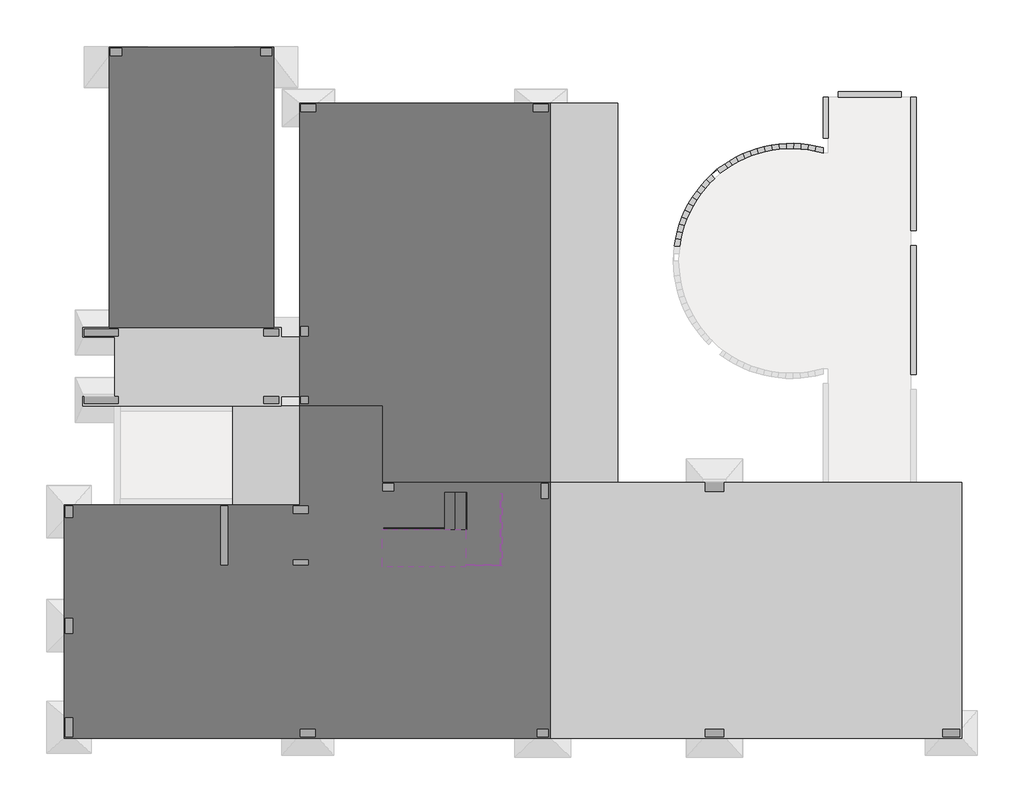
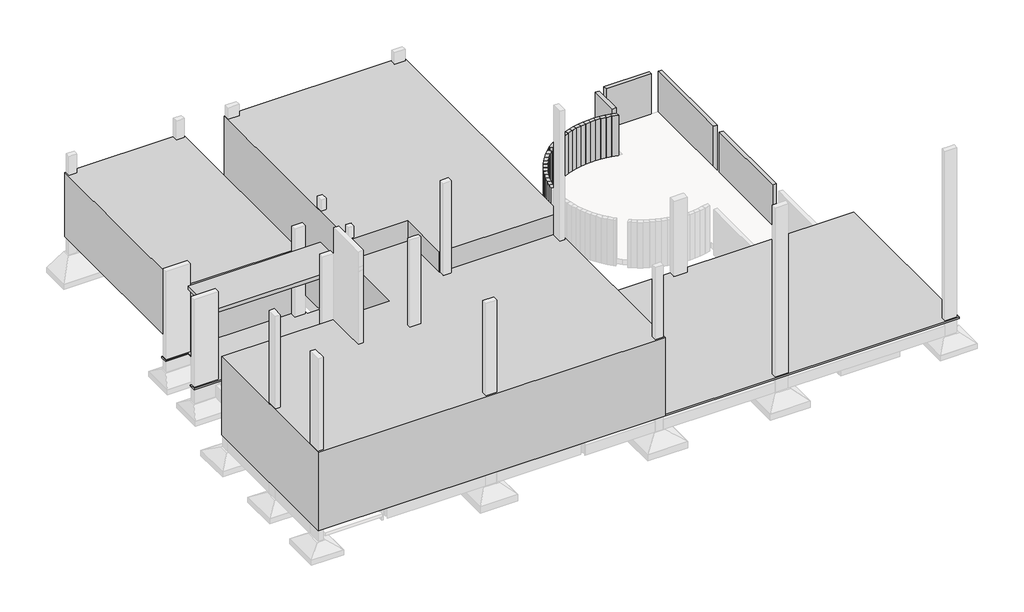
# One storey, part 4 of 4: 29 beams, 7 proxies, 6 railings, 2 stair flights, 1 slab.
# Revit data of these elements (continued)
# Type "ML_Guarda_corpo lance1 : ML_Guarda_corpo lance" (continued)
#   ME_Material Tipo Vidro [instance default] = .VIDRO GENÉRICO
# Element 1 (IfcBeam, "TQS - Viga retangular : 14.0 x 180.0")
#   Uso = "ESTRUTURA"
#   Titulo = "VP1"
#   Chave = "-983"
#   Tipo Elemento = "Viga"
#   SHA1 = "70CFAD44B8F4F6228BE95B7E8E7C3E9A2DD88366"
#   Revisão = ""
#   Tipo de carga = ""
#   Divisor de flexao = ""
#   Secao = ""
#   Configuracao = ""
#   Angulo (graus) = ""
#   Detalhamento = ""
#   Casos de vento manual = ""
#   Tipo = ""
#   Alcas = ""
#   Furos = ""
#   Pino = ""
#   Distribuicao = ""
#   Solidarizado = ""
#   Solidarizar na montagem = ""
#   Unir com o próximo = ""
#   Grupo pre moldado = ""
#   Verificado = ""
#   Concreto C = ""
#   Taxa de armadura (kgf/m³) = 0
#   Carga (tf/m²) = 0
#   Carga (tf/m) = 0
#   Carga (tf) = 0
#   Altura = 1.80 m
#   Rebaixo = 0.15 m
#   Largura = 0.14 m
#   Distancia a face = 0.00 m
#   Distancia ao eixo = 0.00 m
#   Altura gerber esquerda = 0.00 m
#   Largura gerber esquerda = 0.00 m
#   Altura gerber direita = 0.00 m
#   Largura gerber direita = 0.00 m
#   Resultado de Ensaios fck (MPa) = 0
#   Unique TQS ID = -983
#   Principal = yes
#   Structural Material = none
#   Phase Created = CC_AP/ESTR
# Element 2 (IfcBeam, "TQS - Viga retangular : 14.0 x 180.0")
#   Uso = "ESTRUTURA"
#   Titulo = "VP6"
#   Chave = "-1015"
#   Tipo Elemento = "Viga"
#   SHA1 = "4E9806910888EA421A8E9B5F41FC3E19263D6A9E"
#   Revisão = ""
#   Tipo de carga = ""
#   Divisor de flexao = ""
#   Secao = ""
#   Configuracao = ""
#   Angulo (graus) = ""
#   Detalhamento = ""
#   Casos de vento manual = ""
#   Tipo = ""
#   Alcas = ""
#   Furos = ""
#   Pino = ""
#   Distribuicao = ""
#   Solidarizado = ""
#   Solidarizar na montagem = ""
#   Unir com o próximo = ""
#   Grupo pre moldado = ""
#   Verificado = ""
#   Concreto C = ""
#   Taxa de armadura (kgf/m³) = 0
#   Carga (tf/m²) = 0
#   Carga (tf/m) = 0
#   Carga (tf) = 0
#   Altura = 1.80 m
#   Rebaixo = 0.15 m
#   Largura = 0.14 m
#   Distancia a face = 0.00 m
#   Distancia ao eixo = 0.00 m
#   Altura gerber esquerda = 0.00 m
#   Largura gerber esquerda = 0.00 m
#   Altura gerber direita = 0.00 m
#   Largura gerber direita = 0.00 m
#   Resultado de Ensaios fck (MPa) = 0
#   Unique TQS ID = -1015
#   Principal = yes
#   Structural Material = none
#   Phase Created = CC_AP/ESTR
# Element 3 (IfcBeam, "TQS - Viga retangular : 14.0 x 180.0")
#   Uso = "ESTRUTURA"
#   Titulo = "VP6"
#   Chave = "-1016"
#   Tipo Elemento = "Viga"
#   SHA1 = "01F1283C1B0C380DFDB901244E097327FB4B1C7E"
#   Revisão = ""
#   Tipo de carga = ""
#   Divisor de flexao = ""
#   Secao = ""
#   Configuracao = ""
#   Angulo (graus) = ""
#   Detalhamento = ""
#   Casos de vento manual = ""
#   Tipo = ""
#   Alcas = ""
#   Furos = ""
#   Pino = ""
#   Distribuicao = ""
#   Solidarizado = ""
#   Solidarizar na montagem = ""
#   Unir com o próximo = ""
#   Grupo pre moldado = ""
#   Verificado = ""
#   Concreto C = ""
#   Taxa de armadura (kgf/m³) = 0
#   Carga (tf/m²) = 0
#   Carga (tf/m) = 0
#   Carga (tf) = 0
#   Altura = 1.80 m
#   Rebaixo = 0.15 m
#   Largura = 0.14 m
#   Distancia a face = 0.00 m
#   Distancia ao eixo = 0.00 m
#   Altura gerber esquerda = 0.00 m
#   Largura gerber esquerda = 0.00 m
#   Altura gerber direita = 0.00 m
#   Largura gerber direita = 0.00 m
#   Resultado de Ensaios fck (MPa) = 0
#   Unique TQS ID = -1016
#   Principal = yes
#   Structural Material = none
#   Phase Created = CC_AP/ESTR
# Element 4 (IfcBeam, "TQS - Viga retangular : 14.0 x 180.0")
#   Uso = "ESTRUTURA"
#   Titulo = "VP6"
#   Chave = "-1017"
#   Tipo Elemento = "Viga"
#   SHA1 = "22C0BDACD46D49F6E4190D80621E2138C68CD36C"
#   Revisão = ""
#   Tipo de carga = ""
#   Divisor de flexao = ""
#   Secao = ""
#   Configuracao = ""
#   Angulo (graus) = ""
#   Detalhamento = ""
#   Casos de vento manual = ""
#   Tipo = ""
#   Alcas = ""
#   Furos = ""
#   Pino = ""
#   Distribuicao = ""
#   Solidarizado = ""
#   Solidarizar na montagem = ""
#   Unir com o próximo = ""
#   Grupo pre moldado = ""
#   Verificado = ""
#   Concreto C = ""
#   Taxa de armadura (kgf/m³) = 0
#   Carga (tf/m²) = 0
#   Carga (tf/m) = 0
#   Carga (tf) = 0
#   Altura = 1.80 m
#   Rebaixo = 0.15 m
#   Largura = 0.14 m
#   Distancia a face = 0.00 m
#   Distancia ao eixo = 0.00 m
#   Altura gerber esquerda = 0.00 m
#   Largura gerber esquerda = 0.00 m
#   Altura gerber direita = 0.00 m
#   Largura gerber direita = 0.00 m
#   Resultado de Ensaios fck (MPa) = 0
#   Unique TQS ID = -1017
#   Principal = yes
#   Structural Material = none
#   Phase Created = CC_AP/ESTR
# Element 5 (IfcBeam, "TQS - Viga retangular : 14.0 x 180.0")
#   Uso = "ESTRUTURA"
#   Titulo = "VP6"
#   Chave = "-1018"
#   Tipo Elemento = "Viga"
#   SHA1 = "D04A2C827C3C8BC1853343DA7F217DB9B9B2F05D"
#   Revisão = ""
#   Tipo de carga = ""
#   Divisor de flexao = ""
#   Secao = ""
#   Configuracao = ""
#   Angulo (graus) = ""
#   Detalhamento = ""
#   Casos de vento manual = ""
#   Tipo = ""
#   Alcas = ""
#   Furos = ""
#   Pino = ""
#   Distribuicao = ""
#   Solidarizado = ""
#   Solidarizar na montagem = ""
#   Unir com o próximo = ""
#   Grupo pre moldado = ""
#   Verificado = ""
#   Concreto C = ""
#   Taxa de armadura (kgf/m³) = 0
#   Carga (tf/m²) = 0
#   Carga (tf/m) = 0
#   Carga (tf) = 0
#   Altura = 1.80 m
#   Rebaixo = 0.15 m
#   Largura = 0.14 m
#   Distancia a face = 0.00 m
#   Distancia ao eixo = 0.00 m
#   Altura gerber esquerda = 0.00 m
#   Largura gerber esquerda = 0.00 m
#   Altura gerber direita = 0.00 m
#   Largura gerber direita = 0.00 m
#   Resultado de Ensaios fck (MPa) = 0
#   Unique TQS ID = -1018
#   Principal = yes
#   Structural Material = none
#   Phase Created = CC_AP/ESTR
# Element 6 (IfcBeam, "TQS - Viga retangular : 14.0 x 180.0")
#   Uso = "ESTRUTURA"
#   Titulo = "VP6"
#   Chave = "-1019"
#   Tipo Elemento = "Viga"
#   SHA1 = "0D182E2612785E293A5A4969EBA47990CD3E9117"
#   Revisão = ""
#   Tipo de carga = ""
#   Divisor de flexao = ""
#   Secao = ""
#   Configuracao = ""
#   Angulo (graus) = ""
#   Detalhamento = ""
#   Casos de vento manual = ""
#   Tipo = ""
#   Alcas = ""
#   Furos = ""
#   Pino = ""
#   Distribuicao = ""
#   Solidarizado = ""
#   Solidarizar na montagem = ""
#   Unir com o próximo = ""
#   Grupo pre moldado = ""
#   Verificado = ""
#   Concreto C = ""
#   Taxa de armadura (kgf/m³) = 0
#   Carga (tf/m²) = 0
#   Carga (tf/m) = 0
#   Carga (tf) = 0
#   Altura = 1.80 m
#   Rebaixo = 0.15 m
#   Largura = 0.14 m
#   Distancia a face = 0.00 m
#   Distancia ao eixo = 0.00 m
#   Altura gerber esquerda = 0.00 m
#   Largura gerber esquerda = 0.00 m
#   Altura gerber direita = 0.00 m
#   Largura gerber direita = 0.00 m
#   Resultado de Ensaios fck (MPa) = 0
#   Unique TQS ID = -1019
#   Principal = yes
#   Structural Material = none
#   Phase Created = CC_AP/ESTR
# Element 7 (IfcBeam, "TQS - Viga retangular : 14.0 x 180.0")
#   Uso = "ESTRUTURA"
#   Titulo = "VP6"
#   Chave = "-1020"
#   Tipo Elemento = "Viga"
#   SHA1 = "8A5DF36B72EBE22F2A453D6F9BADDE3EA3E2A9B4"
#   Revisão = ""
#   Tipo de carga = ""
#   Divisor de flexao = ""
#   Secao = ""
#   Configuracao = ""
#   Angulo (graus) = ""
#   Detalhamento = ""
#   Casos de vento manual = ""
#   Tipo = ""
#   Alcas = ""
#   Furos = ""
#   Pino = ""
#   Distribuicao = ""
#   Solidarizado = ""
#   Solidarizar na montagem = ""
#   Unir com o próximo = ""
#   Grupo pre moldado = ""
#   Verificado = ""
#   Concreto C = ""
#   Taxa de armadura (kgf/m³) = 0
#   Carga (tf/m²) = 0
#   Carga (tf/m) = 0
#   Carga (tf) = 0
#   Altura = 1.80 m
#   Rebaixo = 0.15 m
#   Largura = 0.14 m
#   Distancia a face = 0.00 m
#   Distancia ao eixo = 0.00 m
#   Altura gerber esquerda = 0.00 m
#   Largura gerber esquerda = 0.00 m
#   Altura gerber direita = 0.00 m
#   Largura gerber direita = 0.00 m
#   Resultado de Ensaios fck (MPa) = 0
#   Unique TQS ID = -1020
#   Principal = yes
#   Structural Material = none
#   Phase Created = CC_AP/ESTR
# Element 8 (IfcBeam, "TQS - Viga retangular : 14.0 x 180.0")
#   Uso = "ESTRUTURA"
#   Titulo = "VP6"
#   Chave = "-1021"
#   Tipo Elemento = "Viga"
#   SHA1 = "E996D88AC41B572457E87FBE2BFAA83C91B590B4"
#   Revisão = ""
#   Tipo de carga = ""
#   Divisor de flexao = ""
#   Secao = ""
#   Configuracao = ""
#   Angulo (graus) = ""
#   Detalhamento = ""
#   Casos de vento manual = ""
#   Tipo = ""
#   Alcas = ""
#   Furos = ""
#   Pino = ""
#   Distribuicao = ""
#   Solidarizado = ""
#   Solidarizar na montagem = ""
#   Unir com o próximo = ""
#   Grupo pre moldado = ""
#   Verificado = ""
#   Concreto C = ""
#   Taxa de armadura (kgf/m³) = 0
#   Carga (tf/m²) = 0
#   Carga (tf/m) = 0
#   Carga (tf) = 0
#   Altura = 1.80 m
#   Rebaixo = 0.15 m
#   Largura = 0.14 m
#   Distancia a face = 0.00 m
#   Distancia ao eixo = 0.00 m
#   Altura gerber esquerda = 0.00 m
#   Largura gerber esquerda = 0.00 m
#   Altura gerber direita = 0.00 m
#   Largura gerber direita = 0.00 m
#   Resultado de Ensaios fck (MPa) = 0
#   Unique TQS ID = -1021
#   Principal = yes
#   Structural Material = none
#   Phase Created = CC_AP/ESTR
# Element 9 (IfcBeam, "TQS - Viga retangular : 14.0 x 180.0")
#   Uso = "ESTRUTURA"
#   Titulo = "VP6"
#   Chave = "-1022"
#   Tipo Elemento = "Viga"
#   SHA1 = "0B33ED0C5CE953F65B7DD0F51C60662F46F82846"
#   Revisão = ""
#   Tipo de carga = ""
#   Divisor de flexao = ""
#   Secao = ""
#   Configuracao = ""
#   Angulo (graus) = ""
#   Detalhamento = ""
#   Casos de vento manual = ""
#   Tipo = ""
#   Alcas = ""
#   Furos = ""
#   Pino = ""
#   Distribuicao = ""
#   Solidarizado = ""
#   Solidarizar na montagem = ""
#   Unir com o próximo = ""
#   Grupo pre moldado = ""
#   Verificado = ""
#   Concreto C = ""
#   Taxa de armadura (kgf/m³) = 0
#   Carga (tf/m²) = 0
#   Carga (tf/m) = 0
#   Carga (tf) = 0
#   Altura = 1.80 m
#   Rebaixo = 0.15 m
#   Largura = 0.14 m
#   Distancia a face = 0.00 m
#   Distancia ao eixo = 0.00 m
#   Altura gerber esquerda = 0.00 m
#   Largura gerber esquerda = 0.00 m
#   Altura gerber direita = 0.00 m
#   Largura gerber direita = 0.00 m
#   Resultado de Ensaios fck (MPa) = 0
#   Unique TQS ID = -1022
#   Principal = yes
#   Structural Material = none
#   Phase Created = CC_AP/ESTR
# Element 10 (IfcBeam, "TQS - Viga retangular : 14.0 x 180.0")
#   Uso = "ESTRUTURA"
#   Titulo = "VP6"
#   Chave = "-1023"
#   Tipo Elemento = "Viga"
#   SHA1 = "7A0208B774D9472BDEB9F4D9C600465610707295"
#   Revisão = ""
#   Tipo de carga = ""
#   Divisor de flexao = ""
#   Secao = ""
#   Configuracao = ""
#   Angulo (graus) = ""
#   Detalhamento = ""
#   Casos de vento manual = ""
#   Tipo = ""
#   Alcas = ""
#   Furos = ""
#   Pino = ""
#   Distribuicao = ""
#   Solidarizado = ""
#   Solidarizar na montagem = ""
#   Unir com o próximo = ""
#   Grupo pre moldado = ""
#   Verificado = ""
#   Concreto C = ""
#   Taxa de armadura (kgf/m³) = 0
#   Carga (tf/m²) = 0
#   Carga (tf/m) = 0
#   Carga (tf) = 0
#   Altura = 1.80 m
#   Rebaixo = 0.15 m
#   Largura = 0.14 m
#   Distancia a face = 0.00 m
#   Distancia ao eixo = 0.00 m
#   Altura gerber esquerda = 0.00 m
#   Largura gerber esquerda = 0.00 m
#   Altura gerber direita = 0.00 m
#   Largura gerber direita = 0.00 m
#   Resultado de Ensaios fck (MPa) = 0
#   Unique TQS ID = -1023
#   Principal = yes
#   Structural Material = none
#   Phase Created = CC_AP/ESTR
# Element 11 (IfcBeam, "TQS - Viga retangular : 14.0 x 180.0")
#   Uso = "ESTRUTURA"
#   Titulo = "VP6"
#   Chave = "-1024"
#   Tipo Elemento = "Viga"
#   SHA1 = "84182F31E964F02A91D7472A67EEC15D959BEA6F"
#   Revisão = ""
#   Tipo de carga = ""
#   Divisor de flexao = ""
#   Secao = ""
#   Configuracao = ""
#   Angulo (graus) = ""
#   Detalhamento = ""
#   Casos de vento manual = ""
#   Tipo = ""
#   Alcas = ""
#   Furos = ""
#   Pino = ""
#   Distribuicao = ""
#   Solidarizado = ""
#   Solidarizar na montagem = ""
#   Unir com o próximo = ""
#   Grupo pre moldado = ""
#   Verificado = ""
#   Concreto C = ""
#   Taxa de armadura (kgf/m³) = 0
#   Carga (tf/m²) = 0
#   Carga (tf/m) = 0
#   Carga (tf) = 0
#   Altura = 1.80 m
#   Rebaixo = 0.15 m
#   Largura = 0.14 m
#   Distancia a face = 0.00 m
#   Distancia ao eixo = 0.00 m
#   Altura gerber esquerda = 0.00 m
#   Largura gerber esquerda = 0.00 m
#   Altura gerber direita = 0.00 m
#   Largura gerber direita = 0.00 m
#   Resultado de Ensaios fck (MPa) = 0
#   Unique TQS ID = -1024
#   Principal = yes
#   Structural Material = none
#   Phase Created = CC_AP/ESTR
# Element 12 (IfcBeam, "TQS - Viga retangular : 14.0 x 180.0")
#   Uso = "ESTRUTURA"
#   Titulo = "VP6"
#   Chave = "-1025"
#   Tipo Elemento = "Viga"
#   SHA1 = "018AD11D8442C61DF0F4C6D5519537CB9DF1785E"
#   Revisão = ""
#   Tipo de carga = ""
#   Divisor de flexao = ""
#   Secao = ""
#   Configuracao = ""
#   Angulo (graus) = ""
#   Detalhamento = ""
#   Casos de vento manual = ""
#   Tipo = ""
#   Alcas = ""
#   Furos = ""
#   Pino = ""
#   Distribuicao = ""
#   Solidarizado = ""
#   Solidarizar na montagem = ""
#   Unir com o próximo = ""
#   Grupo pre moldado = ""
#   Verificado = ""
#   Concreto C = ""
#   Taxa de armadura (kgf/m³) = 0
#   Carga (tf/m²) = 0
#   Carga (tf/m) = 0
#   Carga (tf) = 0
#   Altura = 1.80 m
#   Rebaixo = 0.15 m
#   Largura = 0.14 m
#   Distancia a face = 0.00 m
#   Distancia ao eixo = 0.00 m
#   Altura gerber esquerda = 0.00 m
#   Largura gerber esquerda = 0.00 m
#   Altura gerber direita = 0.00 m
#   Largura gerber direita = 0.00 m
#   Resultado de Ensaios fck (MPa) = 0
#   Unique TQS ID = -1025
#   Principal = yes
#   Structural Material = none
#   Phase Created = CC_AP/ESTR
# Element 13 (IfcBeam, "TQS - Viga retangular : 14.0 x 180.0")
#   Uso = "ESTRUTURA"
#   Titulo = "VP7"
#   Chave = "-1026"
#   Tipo Elemento = "Viga"
#   SHA1 = "EE0903180FC4F74752EE8D351596400DB6C4E3D3"
#   Revisão = ""
#   Tipo de carga = ""
#   Divisor de flexao = ""
#   Secao = ""
#   Configuracao = ""
#   Angulo (graus) = ""
#   Detalhamento = ""
#   Casos de vento manual = ""
#   Tipo = ""
#   Alcas = ""
#   Furos = ""
#   Pino = ""
#   Distribuicao = ""
#   Solidarizado = ""
#   Solidarizar na montagem = ""
#   Unir com o próximo = ""
#   Grupo pre moldado = ""
#   Verificado = ""
#   Concreto C = ""
#   Taxa de armadura (kgf/m³) = 0
#   Carga (tf/m²) = 0
#   Carga (tf/m) = 0
#   Carga (tf) = 0
#   Altura = 1.80 m
#   Rebaixo = 0.15 m
#   Largura = 0.14 m
#   Distancia a face = 0.00 m
#   Distancia ao eixo = 0.00 m
#   Altura gerber esquerda = 0.00 m
#   Largura gerber esquerda = 0.00 m
#   Altura gerber direita = 0.00 m
#   Largura gerber direita = 0.00 m
#   Resultado de Ensaios fck (MPa) = 0
#   Unique TQS ID = -1026
#   Principal = yes
#   Structural Material = none
#   Phase Created = CC_AP/ESTR
# Element 14 (IfcBeam, "TQS - Viga retangular : 14.0 x 180.0")
#   Uso = "ESTRUTURA"
#   Titulo = "VP7"
#   Chave = "-1027"
#   Tipo Elemento = "Viga"
#   SHA1 = "9C0E264E63AB224DB050780EBEBCCF0090D66D0A"
#   Revisão = ""
#   Tipo de carga = ""
#   Divisor de flexao = ""
#   Secao = ""
#   Configuracao = ""
#   Angulo (graus) = ""
#   Detalhamento = ""
#   Casos de vento manual = ""
#   Tipo = ""
#   Alcas = ""
#   Furos = ""
#   Pino = ""
#   Distribuicao = ""
#   Solidarizado = ""
#   Solidarizar na montagem = ""
#   Unir com o próximo = ""
#   Grupo pre moldado = ""
#   Verificado = ""
#   Concreto C = ""
#   Taxa de armadura (kgf/m³) = 0
#   Carga (tf/m²) = 0
#   Carga (tf/m) = 0
#   Carga (tf) = 0
#   Altura = 1.80 m
#   Rebaixo = 0.15 m
#   Largura = 0.14 m
#   Distancia a face = 0.00 m
#   Distancia ao eixo = 0.00 m
#   Altura gerber esquerda = 0.00 m
#   Largura gerber esquerda = 0.00 m
#   Altura gerber direita = 0.00 m
#   Largura gerber direita = 0.00 m
#   Resultado de Ensaios fck (MPa) = 0
#   Unique TQS ID = -1027
#   Principal = yes
#   Structural Material = none
#   Phase Created = CC_AP/ESTR
# Element 15 (IfcBeam, "TQS - Viga retangular : 14.0 x 180.0")
#   Uso = "ESTRUTURA"
#   Titulo = "VP7"
#   Chave = "-1028"
#   Tipo Elemento = "Viga"
#   SHA1 = "6E997BB4E590CA8C89FDA8B6D3FF6154DFE7002F"
#   Revisão = ""
#   Tipo de carga = ""
#   Divisor de flexao = ""
#   Secao = ""
#   Configuracao = ""
#   Angulo (graus) = ""
#   Detalhamento = ""
#   Casos de vento manual = ""
#   Tipo = ""
#   Alcas = ""
#   Furos = ""
#   Pino = ""
#   Distribuicao = ""
#   Solidarizado = ""
#   Solidarizar na montagem = ""
#   Unir com o próximo = ""
#   Grupo pre moldado = ""
#   Verificado = ""
#   Concreto C = ""
#   Taxa de armadura (kgf/m³) = 0
#   Carga (tf/m²) = 0
#   Carga (tf/m) = 0
#   Carga (tf) = 0
#   Altura = 1.80 m
#   Rebaixo = 0.15 m
#   Largura = 0.14 m
#   Distancia a face = 0.00 m
#   Distancia ao eixo = 0.00 m
#   Altura gerber esquerda = 0.00 m
#   Largura gerber esquerda = 0.00 m
#   Altura gerber direita = 0.00 m
#   Largura gerber direita = 0.00 m
#   Resultado de Ensaios fck (MPa) = 0
#   Unique TQS ID = -1028
#   Principal = yes
#   Structural Material = none
#   Phase Created = CC_AP/ESTR
# Element 16 (IfcBeam, "TQS - Viga retangular : 14.0 x 180.0")
#   Uso = "ESTRUTURA"
#   Titulo = "VP7"
#   Chave = "-1029"
#   Tipo Elemento = "Viga"
#   SHA1 = "7DDF74561A6D880C43286526A234CDA9ECB81B66"
#   Revisão = ""
#   Tipo de carga = ""
#   Divisor de flexao = ""
#   Secao = ""
#   Configuracao = ""
#   Angulo (graus) = ""
#   Detalhamento = ""
#   Casos de vento manual = ""
#   Tipo = ""
#   Alcas = ""
#   Furos = ""
#   Pino = ""
#   Distribuicao = ""
#   Solidarizado = ""
#   Solidarizar na montagem = ""
#   Unir com o próximo = ""
#   Grupo pre moldado = ""
#   Verificado = ""
#   Concreto C = ""
#   Taxa de armadura (kgf/m³) = 0
#   Carga (tf/m²) = 0
#   Carga (tf/m) = 0
#   Carga (tf) = 0
#   Altura = 1.80 m
#   Rebaixo = 0.15 m
#   Largura = 0.14 m
#   Distancia a face = 0.00 m
#   Distancia ao eixo = 0.00 m
#   Altura gerber esquerda = 0.00 m
#   Largura gerber esquerda = 0.00 m
#   Altura gerber direita = 0.00 m
#   Largura gerber direita = 0.00 m
#   Resultado de Ensaios fck (MPa) = 0
#   Unique TQS ID = -1029
#   Principal = yes
#   Structural Material = none
#   Phase Created = CC_AP/ESTR
# Element 17 (IfcBeam, "TQS - Viga retangular : 14.0 x 180.0")
#   Uso = "ESTRUTURA"
#   Titulo = "VP7"
#   Chave = "-1030"
#   Tipo Elemento = "Viga"
#   SHA1 = "2D411C14CB7CE55D4F1E0A23351751B1C30F9CC4"
#   Revisão = ""
#   Tipo de carga = ""
#   Divisor de flexao = ""
#   Secao = ""
#   Configuracao = ""
#   Angulo (graus) = ""
#   Detalhamento = ""
#   Casos de vento manual = ""
#   Tipo = ""
#   Alcas = ""
#   Furos = ""
#   Pino = ""
#   Distribuicao = ""
#   Solidarizado = ""
#   Solidarizar na montagem = ""
#   Unir com o próximo = ""
#   Grupo pre moldado = ""
#   Verificado = ""
#   Concreto C = ""
#   Taxa de armadura (kgf/m³) = 0
#   Carga (tf/m²) = 0
#   Carga (tf/m) = 0
#   Carga (tf) = 0
#   Altura = 1.80 m
#   Rebaixo = 0.15 m
#   Largura = 0.14 m
#   Distancia a face = 0.00 m
#   Distancia ao eixo = 0.00 m
#   Altura gerber esquerda = 0.00 m
#   Largura gerber esquerda = 0.00 m
#   Altura gerber direita = 0.00 m
#   Largura gerber direita = 0.00 m
#   Resultado de Ensaios fck (MPa) = 0
#   Unique TQS ID = -1030
#   Principal = yes
#   Structural Material = none
#   Phase Created = CC_AP/ESTR
# Element 18 (IfcBeam, "TQS - Viga retangular : 14.0 x 180.0")
#   Uso = "ESTRUTURA"
#   Titulo = "VP7"
#   Chave = "-1031"
#   Tipo Elemento = "Viga"
#   SHA1 = "171049F04C5F75504E61353FF9C8DE909D3AD5A1"
#   Revisão = ""
#   Tipo de carga = ""
#   Divisor de flexao = ""
#   Secao = ""
#   Configuracao = ""
#   Angulo (graus) = ""
#   Detalhamento = ""
#   Casos de vento manual = ""
#   Tipo = ""
#   Alcas = ""
#   Furos = ""
#   Pino = ""
#   Distribuicao = ""
#   Solidarizado = ""
#   Solidarizar na montagem = ""
#   Unir com o próximo = ""
#   Grupo pre moldado = ""
#   Verificado = ""
#   Concreto C = ""
#   Taxa de armadura (kgf/m³) = 0
#   Carga (tf/m²) = 0
#   Carga (tf/m) = 0
#   Carga (tf) = 0
#   Altura = 1.80 m
#   Rebaixo = 0.15 m
#   Largura = 0.14 m
#   Distancia a face = 0.00 m
#   Distancia ao eixo = 0.00 m
#   Altura gerber esquerda = 0.00 m
#   Largura gerber esquerda = 0.00 m
#   Altura gerber direita = 0.00 m
#   Largura gerber direita = 0.00 m
#   Resultado de Ensaios fck (MPa) = 0
#   Unique TQS ID = -1031
#   Principal = yes
#   Structural Material = none
#   Phase Created = CC_AP/ESTR
# Element 19 (IfcBeam, "TQS - Viga retangular : 14.0 x 180.0")
#   Uso = "ESTRUTURA"
#   Titulo = "VP7"
#   Chave = "-1032"
#   Tipo Elemento = "Viga"
#   SHA1 = "6DF824D13F17D5A6128940B40DFD1C2714CD6B1E"
#   Revisão = ""
#   Tipo de carga = ""
#   Divisor de flexao = ""
#   Secao = ""
#   Configuracao = ""
#   Angulo (graus) = ""
#   Detalhamento = ""
#   Casos de vento manual = ""
#   Tipo = ""
#   Alcas = ""
#   Furos = ""
#   Pino = ""
#   Distribuicao = ""
#   Solidarizado = ""
#   Solidarizar na montagem = ""
#   Unir com o próximo = ""
#   Grupo pre moldado = ""
#   Verificado = ""
#   Concreto C = ""
#   Taxa de armadura (kgf/m³) = 0
#   Carga (tf/m²) = 0
#   Carga (tf/m) = 0
#   Carga (tf) = 0
#   Altura = 1.80 m
#   Rebaixo = 0.15 m
#   Largura = 0.14 m
#   Distancia a face = 0.00 m
#   Distancia ao eixo = 0.00 m
#   Altura gerber esquerda = 0.00 m
#   Largura gerber esquerda = 0.00 m
#   Altura gerber direita = 0.00 m
#   Largura gerber direita = 0.00 m
#   Resultado de Ensaios fck (MPa) = 0
#   Unique TQS ID = -1032
#   Principal = yes
#   Structural Material = none
#   Phase Created = CC_AP/ESTR
# Element 20 (IfcBeam, "TQS - Viga retangular : 14.0 x 180.0")
#   Uso = "ESTRUTURA"
#   Titulo = "VP7"
#   Chave = "-1033"
#   Tipo Elemento = "Viga"
#   SHA1 = "2A35CBBA7314E7981D7057AA3DC248078908D855"
#   Revisão = ""
#   Tipo de carga = ""
#   Divisor de flexao = ""
#   Secao = ""
#   Configuracao = ""
#   Angulo (graus) = ""
#   Detalhamento = ""
#   Casos de vento manual = ""
#   Tipo = ""
#   Alcas = ""
#   Furos = ""
#   Pino = ""
#   Distribuicao = ""
#   Solidarizado = ""
#   Solidarizar na montagem = ""
#   Unir com o próximo = ""
#   Grupo pre moldado = ""
#   Verificado = ""
#   Concreto C = ""
#   Taxa de armadura (kgf/m³) = 0
#   Carga (tf/m²) = 0
#   Carga (tf/m) = 0
#   Carga (tf) = 0
#   Altura = 1.80 m
#   Rebaixo = 0.15 m
#   Largura = 0.14 m
#   Distancia a face = 0.00 m
#   Distancia ao eixo = 0.00 m
#   Altura gerber esquerda = 0.00 m
#   Largura gerber esquerda = 0.00 m
#   Altura gerber direita = 0.00 m
#   Largura gerber direita = 0.00 m
#   Resultado de Ensaios fck (MPa) = 0
#   Unique TQS ID = -1033
#   Principal = yes
#   Structural Material = none
#   Phase Created = CC_AP/ESTR
# Element 21 (IfcBeam, "TQS - Viga retangular : 14.0 x 180.0")
#   Uso = "ESTRUTURA"
#   Titulo = "VP7"
#   Chave = "-1034"
#   Tipo Elemento = "Viga"
#   SHA1 = "2B52F4D055F474E9CD7666D6686E78183A6E7EC4"
#   Revisão = ""
#   Tipo de carga = ""
#   Divisor de flexao = ""
#   Secao = ""
#   Configuracao = ""
#   Angulo (graus) = ""
#   Detalhamento = ""
#   Casos de vento manual = ""
#   Tipo = ""
#   Alcas = ""
#   Furos = ""
#   Pino = ""
#   Distribuicao = ""
#   Solidarizado = ""
#   Solidarizar na montagem = ""
#   Unir com o próximo = ""
#   Grupo pre moldado = ""
#   Verificado = ""
#   Concreto C = ""
#   Taxa de armadura (kgf/m³) = 0
#   Carga (tf/m²) = 0
#   Carga (tf/m) = 0
#   Carga (tf) = 0
#   Altura = 1.80 m
#   Rebaixo = 0.15 m
#   Largura = 0.14 m
#   Distancia a face = 0.00 m
#   Distancia ao eixo = 0.00 m
#   Altura gerber esquerda = 0.00 m
#   Largura gerber esquerda = 0.00 m
#   Altura gerber direita = 0.00 m
#   Largura gerber direita = 0.00 m
#   Resultado de Ensaios fck (MPa) = 0
#   Unique TQS ID = -1034
#   Principal = yes
#   Structural Material = none
#   Phase Created = CC_AP/ESTR
# Element 22 (IfcBeam, "TQS - Viga retangular : 14.0 x 180.0")
#   Uso = "ESTRUTURA"
#   Titulo = "VP7"
#   Chave = "-1035"
#   Tipo Elemento = "Viga"
#   SHA1 = "4164F1A2AAB45DB19362C3FEFBBEE02BFBC2F3D5"
#   Revisão = ""
#   Tipo de carga = ""
#   Divisor de flexao = ""
#   Secao = ""
#   Configuracao = ""
#   Angulo (graus) = ""
#   Detalhamento = ""
#   Casos de vento manual = ""
#   Tipo = ""
#   Alcas = ""
#   Furos = ""
#   Pino = ""
#   Distribuicao = ""
#   Solidarizado = ""
#   Solidarizar na montagem = ""
#   Unir com o próximo = ""
#   Grupo pre moldado = ""
#   Verificado = ""
#   Concreto C = ""
#   Taxa de armadura (kgf/m³) = 0
#   Carga (tf/m²) = 0
#   Carga (tf/m) = 0
#   Carga (tf) = 0
#   Altura = 1.80 m
#   Rebaixo = 0.15 m
#   Largura = 0.14 m
#   Distancia a face = 0.00 m
#   Distancia ao eixo = 0.00 m
#   Altura gerber esquerda = 0.00 m
#   Largura gerber esquerda = 0.00 m
#   Altura gerber direita = 0.00 m
#   Largura gerber direita = 0.00 m
#   Resultado de Ensaios fck (MPa) = 0
#   Unique TQS ID = -1035
#   Principal = yes
#   Structural Material = none
#   Phase Created = CC_AP/ESTR
# Element 23 (IfcBeam, "TQS - Viga retangular : 14.0 x 180.0")
#   Uso = "ESTRUTURA"
#   Titulo = "VP7"
#   Chave = "-1036"
#   Tipo Elemento = "Viga"
#   SHA1 = "488CD87153485AFAB4498525AFF36ABFE92E7622"
#   Revisão = ""
#   Tipo de carga = ""
#   Divisor de flexao = ""
#   Secao = ""
#   Configuracao = ""
#   Angulo (graus) = ""
#   Detalhamento = ""
#   Casos de vento manual = ""
#   Tipo = ""
#   Alcas = ""
#   Furos = ""
#   Pino = ""
#   Distribuicao = ""
#   Solidarizado = ""
#   Solidarizar na montagem = ""
#   Unir com o próximo = ""
#   Grupo pre moldado = ""
#   Verificado = ""
#   Concreto C = ""
#   Taxa de armadura (kgf/m³) = 0
#   Carga (tf/m²) = 0
#   Carga (tf/m) = 0
#   Carga (tf) = 0
#   Altura = 1.80 m
#   Rebaixo = 0.15 m
#   Largura = 0.14 m
#   Distancia a face = 0.00 m
#   Distancia ao eixo = 0.00 m
#   Altura gerber esquerda = 0.00 m
#   Largura gerber esquerda = 0.00 m
#   Altura gerber direita = 0.00 m
#   Largura gerber direita = 0.00 m
#   Resultado de Ensaios fck (MPa) = 0
#   Unique TQS ID = -1036
#   Principal = yes
#   Structural Material = none
#   Phase Created = CC_AP/ESTR
# Element 24 (IfcBeam, "TQS - Viga retangular : 14.0 x 180.0")
#   Uso = "ESTRUTURA"
#   Titulo = "VP7"
#   Chave = "-1037"
#   Tipo Elemento = "Viga"
#   SHA1 = "197F68BC870D688E0A2EC9FD05BD8B81B3EE2891"
#   Revisão = ""
#   Tipo de carga = ""
#   Divisor de flexao = ""
#   Secao = ""
#   Configuracao = ""
#   Angulo (graus) = ""
#   Detalhamento = ""
#   Casos de vento manual = ""
#   Tipo = ""
#   Alcas = ""
#   Furos = ""
#   Pino = ""
#   Distribuicao = ""
#   Solidarizado = ""
#   Solidarizar na montagem = ""
#   Unir com o próximo = ""
#   Grupo pre moldado = ""
#   Verificado = ""
#   Concreto C = ""
#   Taxa de armadura (kgf/m³) = 0
#   Carga (tf/m²) = 0
#   Carga (tf/m) = 0
#   Carga (tf) = 0
#   Altura = 1.80 m
#   Rebaixo = 0.15 m
#   Largura = 0.14 m
#   Distancia a face = 0.00 m
#   Distancia ao eixo = 0.00 m
#   Altura gerber esquerda = 0.00 m
#   Largura gerber esquerda = 0.00 m
#   Altura gerber direita = 0.00 m
#   Largura gerber direita = 0.00 m
#   Resultado de Ensaios fck (MPa) = 0
#   Unique TQS ID = -1037
#   Principal = yes
#   Structural Material = none
#   Phase Created = CC_AP/ESTR
# Element 25 (IfcBeam, "TQS - Viga retangular : 14.0 x 180.0")
#   Uso = "ESTRUTURA"
#   Titulo = "VP7"
#   Chave = "-1038"
#   Tipo Elemento = "Viga"
#   SHA1 = "A01B41D9FF886BEAE3E617D97EE3619056D0B1F6"
#   Revisão = ""
#   Tipo de carga = ""
#   Divisor de flexao = ""
#   Secao = ""
#   Configuracao = ""
#   Angulo (graus) = ""
#   Detalhamento = ""
#   Casos de vento manual = ""
#   Tipo = ""
#   Alcas = ""
#   Furos = ""
#   Pino = ""
#   Distribuicao = ""
#   Solidarizado = ""
#   Solidarizar na montagem = ""
#   Unir com o próximo = ""
#   Grupo pre moldado = ""
#   Verificado = ""
#   Concreto C = ""
#   Taxa de armadura (kgf/m³) = 0
#   Carga (tf/m²) = 0
#   Carga (tf/m) = 0
#   Carga (tf) = 0
#   Altura = 1.80 m
#   Rebaixo = 0.15 m
#   Largura = 0.14 m
#   Distancia a face = 0.00 m
#   Distancia ao eixo = 0.00 m
#   Altura gerber esquerda = 0.00 m
#   Largura gerber esquerda = 0.00 m
#   Altura gerber direita = 0.00 m
#   Largura gerber direita = 0.00 m
#   Resultado de Ensaios fck (MPa) = 0
#   Unique TQS ID = -1038
#   Principal = yes
#   Structural Material = none
#   Phase Created = CC_AP/ESTR
# Element 26 (IfcBeam, "TQS - Viga retangular : 14.0 x 180.0")
#   Uso = "ESTRUTURA"
#   Titulo = "VP7"
#   Chave = "-1039"
#   Tipo Elemento = "Viga"
#   SHA1 = "464C06C93C140F0D2F14A56FBCB9B233FA9BCEFA"
#   Revisão = ""
#   Tipo de carga = ""
#   Divisor de flexao = ""
#   Secao = ""
#   Configuracao = ""
#   Angulo (graus) = ""
#   Detalhamento = ""
#   Casos de vento manual = ""
#   Tipo = ""
#   Alcas = ""
#   Furos = ""
#   Pino = ""
#   Distribuicao = ""
#   Solidarizado = ""
#   Solidarizar na montagem = ""
#   Unir com o próximo = ""
#   Grupo pre moldado = ""
#   Verificado = ""
#   Concreto C = ""
#   Taxa de armadura (kgf/m³) = 0
#   Carga (tf/m²) = 0
#   Carga (tf/m) = 0
#   Carga (tf) = 0
#   Altura = 1.80 m
#   Rebaixo = 0.15 m
#   Largura = 0.14 m
#   Distancia a face = 0.00 m
#   Distancia ao eixo = 0.00 m
#   Altura gerber esquerda = 0.00 m
#   Largura gerber esquerda = 0.00 m
#   Altura gerber direita = 0.00 m
#   Largura gerber direita = 0.00 m
#   Resultado de Ensaios fck (MPa) = 0
#   Unique TQS ID = -1039
#   Principal = yes
#   Structural Material = none
#   Phase Created = CC_AP/ESTR
# Element 27 (IfcBeam, "TQS - Viga retangular : 14.0 x 180.0")
#   Uso = "ESTRUTURA"
#   Titulo = "VP7"
#   Chave = "-1040"
#   Tipo Elemento = "Viga"
#   SHA1 = "4C21DE7F9DAC405A6DCBFB549F747162CD869074"
#   Revisão = ""
#   Tipo de carga = ""
#   Divisor de flexao = ""
#   Secao = ""
#   Configuracao = ""
#   Angulo (graus) = ""
#   Detalhamento = ""
#   Casos de vento manual = ""
#   Tipo = ""
#   Alcas = ""
#   Furos = ""
#   Pino = ""
#   Distribuicao = ""
#   Solidarizado = ""
#   Solidarizar na montagem = ""
#   Unir com o próximo = ""
#   Grupo pre moldado = ""
#   Verificado = ""
#   Concreto C = ""
#   Taxa de armadura (kgf/m³) = 0
#   Carga (tf/m²) = 0
#   Carga (tf/m) = 0
#   Carga (tf) = 0
#   Altura = 1.80 m
#   Rebaixo = 0.15 m
#   Largura = 0.14 m
#   Distancia a face = 0.00 m
#   Distancia ao eixo = 0.00 m
#   Altura gerber esquerda = 0.00 m
#   Largura gerber esquerda = 0.00 m
#   Altura gerber direita = 0.00 m
#   Largura gerber direita = 0.00 m
#   Resultado de Ensaios fck (MPa) = 0
#   Unique TQS ID = -1040
#   Principal = yes
#   Structural Material = none
#   Phase Created = CC_AP/ESTR
# Element 28 (IfcBeam, "TQS - Viga retangular : 14.0 x 180.0")
#   Uso = "ESTRUTURA"
#   Titulo = "VP8"
#   Chave = "-1041"
#   Tipo Elemento = "Viga"
#   SHA1 = "6AA3E4511FE5BFB69BE90AF5BC0D9228BA1EC532"
#   Revisão = ""
#   Tipo de carga = ""
#   Divisor de flexao = ""
#   Secao = ""
#   Configuracao = ""
#   Angulo (graus) = ""
#   Detalhamento = ""
#   Casos de vento manual = ""
#   Tipo = ""
#   Alcas = ""
#   Furos = ""
#   Pino = ""
#   Distribuicao = ""
#   Solidarizado = ""
#   Solidarizar na montagem = ""
#   Unir com o próximo = ""
#   Grupo pre moldado = ""
#   Verificado = ""
#   Concreto C = ""
#   Taxa de armadura (kgf/m³) = 0
#   Carga (tf/m²) = 0
#   Carga (tf/m) = 0
#   Carga (tf) = 0
#   Altura = 1.80 m
#   Rebaixo = 0.15 m
#   Largura = 0.14 m
#   Distancia a face = 0.00 m
#   Distancia ao eixo = 0.00 m
#   Altura gerber esquerda = 0.00 m
#   Largura gerber esquerda = 0.00 m
#   Altura gerber direita = 0.00 m
#   Largura gerber direita = 0.00 m
#   Resultado de Ensaios fck (MPa) = 0
#   Unique TQS ID = -1041
#   Principal = yes
#   Structural Material = none
#   Phase Created = CC_AP/ESTR
# Element 29 (IfcBeam, "TQS - Viga retangular : 14.0 x 180.0")
#   Uso = "ESTRUTURA"
#   Titulo = "VP10"
#   Chave = "-1044"
#   Tipo Elemento = "Viga"
#   SHA1 = "7E9D2D7EE297E45D169793BFEC03634A2C078807"
#   Revisão = ""
#   Tipo de carga = ""
#   Divisor de flexao = ""
#   Secao = ""
#   Configuracao = ""
#   Angulo (graus) = ""
#   Detalhamento = ""
#   Casos de vento manual = ""
#   Tipo = ""
#   Alcas = ""
#   Furos = ""
#   Pino = ""
#   Distribuicao = ""
#   Solidarizado = ""
#   Solidarizar na montagem = ""
#   Unir com o próximo = ""
#   Grupo pre moldado = ""
#   Verificado = ""
#   Concreto C = ""
#   Taxa de armadura (kgf/m³) = 0
#   Carga (tf/m²) = 0
#   Carga (tf/m) = 0
#   Carga (tf) = 0
#   Altura = 1.80 m
#   Rebaixo = 0.15 m
#   Largura = 0.14 m
#   Distancia a face = 0.00 m
#   Distancia ao eixo = 0.00 m
#   Altura gerber esquerda = 0.00 m
#   Largura gerber esquerda = 0.00 m
#   Altura gerber direita = 0.00 m
#   Largura gerber direita = 0.00 m
#   Resultado de Ensaios fck (MPa) = 0
#   Unique TQS ID = -1044
#   Principal = yes
#   Structural Material = none
#   Phase Created = CC_AP/ESTR
# Element 30 (IfcBuildingElementProxy, "GARAGEM : GARAGEM")
#   Phase Created = CC_EV
#   Materials on its faces: "Forma padrão"
# Element 31 (IfcBuildingElementProxy, "PERGOLADO SALAS : PERGOLADO SALAS")
#   Phase Created = CC_EV
#   Materials on its faces: "Forma padrão"
# Element 32 (IfcBuildingElementProxy, "VARANDA GOURMET : VARANDA GOURMET")
#   Phase Created = CC_EV
#   Materials on its faces: "Forma padrão"
# Element 33 (IfcBuildingElementProxy, "PÓRTICO ENTRADA : PÓRTICO ENTRADA")
#   Phase Created = CC_EV
#   Materials on its faces: "Forma padrão"
# Element 34 (IfcBuildingElementProxy, "SALAS : SALAS")
#   Phase Created = CC_EV
#   Materials on its faces: "Forma padrão"
# Element 35 (IfcBuildingElementProxy, "PROJEÇÃO : PROJEÇÃO")
#   Phase Created = CC_EV
#   Materials on its faces: "Forma padrão"
# Element 36 (IfcBuildingElementProxy, "COZINHA E LAVANDERIA : COZINHA E LAVANDERIA")
#   Phase Created = CC_EV
#   Materials on its faces: "Forma padrão"
# Element 37 (IfcRailing, "ML_Perfil U de embutir3 : ML_Perfil U de embutir")
#   Uso = "PATAMAR"
#   ME_Compr = 1.94 m
#   ME_Material Perfil = .ALUMÍNIO COM PINTURA ELETROSTÁTICA BRANCA
#   Phase Created = CC_AP
#   Materials on its faces: ".ALUMÍNIO COM PINTURA ELETROSTÁTICA BRANCA"
# Element 38 (IfcRailing, "ML_Painéis3 : ML_Painéis")
#   Uso = "PATAMAR"
#   ME_Área = 2.1296 m²
#   ME_Espessura = 0.012 m
#   ME_Dist Painéis = 0.002 m
#   ME_Compr Painéis = 1.936 m
#   ME_Compr = 1.94 m
#   ME_Altura = 1.10 m
#   ME_Quant Painéis = 3
#   ME_Painel Único = yes
#   ME_Paineis Vários = no
#   ME_Material Tipo Vidro = .VIDRO GENÉRICO
#   Phase Created = CC_AP
#   Materials on its faces: ".VIDRO GENÉRICO"
# Element 39 (IfcRailing, "ML_Perfil U de embutir4 : ML_Perfil U de embutir")
#   Uso = "PATAMAR"
#   ME_Compr = 0.925 m
#   ME_Material Perfil = .ALUMÍNIO COM PINTURA ELETROSTÁTICA BRANCA
#   Phase Created = CC_AP
#   Materials on its faces: ".ALUMÍNIO COM PINTURA ELETROSTÁTICA BRANCA"
# Element 40 (IfcRailing, "ML_Painéis4 : ML_Painéis")
#   Uso = "PATAMAR"
#   ME_Área = 1.0131 m²
#   ME_Espessura = 0.012 m
#   ME_Dist Painéis = 0.002 m
#   ME_Compr Painéis = 0.921 m
#   ME_Compr = 0.925 m
#   ME_Altura = 1.10 m
#   ME_Quant Painéis = 3
#   ME_Painel Único = yes
#   ME_Paineis Vários = no
#   ME_Material Tipo Vidro = .VIDRO GENÉRICO
#   Phase Created = CC_AP
#   Materials on its faces: ".VIDRO GENÉRICO"
# Element 41 (IfcRailing, "ML_Guarda_corpo lance : ML_Guarda_corpo lance")
#   Uso = "LANCE"
#   ME_Espessura = 0.012 m
#   ME_Material Tipo Vidro = .VIDRO GENÉRICO
#   Phase Created = CC_AP
#   Materials on its faces: ".VIDRO GENÉRICO"
# Element 42 (IfcRailing, "ML_Guarda_corpo lance1 : ML_Guarda_corpo lance")
#   Uso = "LANCE"
#   ME_Espessura = 0.012 m
#   ME_Material Tipo Vidro = .VIDRO GENÉRICO
#   Phase Created = CC_AP
#   Materials on its faces: ".VIDRO GENÉRICO"
# Element 43 (IfcSlab, "Espessura de 300 mm")
#   Phase Created = CC_AP
#   Materials on its faces: ".SOLEIRA DE CUMARÚ"
# Elements 44, 45 (IfcStairFlight, "Profundidade de 150 mm - SEM BOCEL")
#   Phase Created = CC_AP
#   Materials on its faces: ".SOLEIRA DE CUMARÚ", ".CONCRETO ESTRUTURAL"
# Materials
#   ".ALUMÍNIO COM PINTURA ELETROSTÁTICA BRANCA": class "CC_METAIS", colour RGB 241 241 241, transparency 0, Cost = 0
#   ".VIDRO GENÉRICO": class ".CC_VIDRO", colour RGB 0 128 192, transparency 0.9, Description = "Vidro comum", Cost = 0
#   "Forma padrão": class "Genérico", colour RGB 185 189 196, transparency 0.5, Cost = 0
#   ".SOLEIRA DE CUMARÚ": class ".CC_MADEIRAS", colour RGB 188 160 135, transparency 0, Cost = 0
#   ".CONCRETO ESTRUTURAL": class ".CC_CONCRETO", colour RGB 192 192 192, transparency 0, Description = "Concreto moldado no local", Cost = 0
